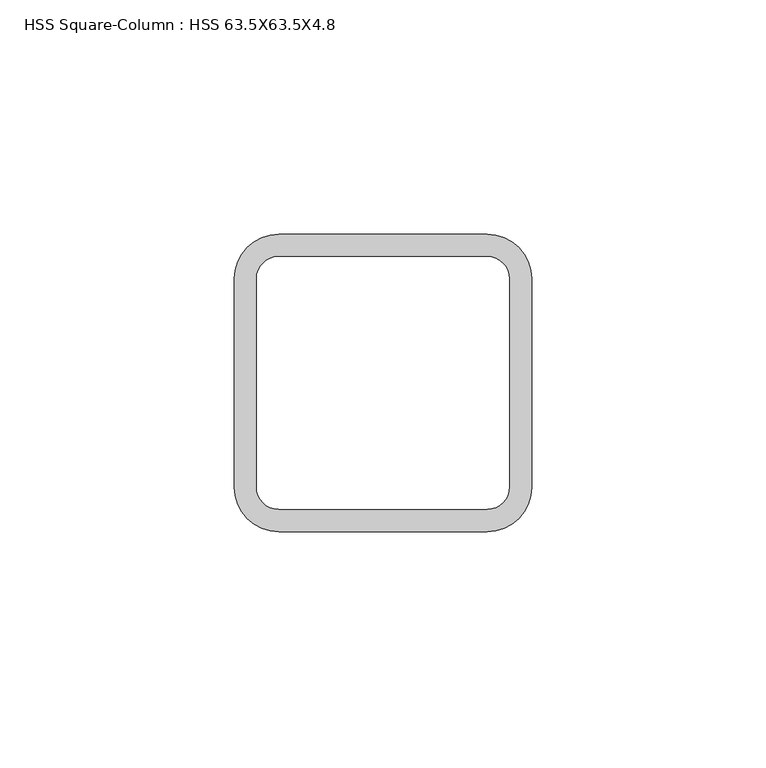
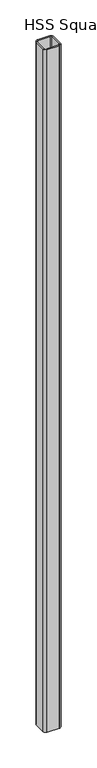
"""IFC4 building model written with IfcOpenShell, lengths in millimetres: column geometry, HSS Square-Column : HSS 63.5X63.5X4.8."""

from ifc_helpers import new_model, si_unit, point, frame, frame_2d, origin, place, context, project, spatial, polyline, circle_curve, trimmed, segment, composite_curve, outline, extrude, source, transform, mapped, element, save


def hss_square_column_hss_63_5x63_5x4_8_397be378(model_context):
    return source(origin(), model_context, "Body", "SweptSolid", [
        extrude(outline(composite_curve([segment(trimmed(circle_curve(frame_2d((22.225, 22.225)), 9.525), [point((22.225, 31.75))], [point((31.75, 22.225))], False, "CARTESIAN"), True, "CONTINUOUS"), segment(polyline([(31.75, 22.225), (31.75, -22.225)]), True, "CONTINUOUS"), segment(trimmed(circle_curve(frame_2d((22.225, -22.225)), 9.525), [point((31.75, -22.225))], [point((22.225, -31.75))], False, "CARTESIAN"), True, "CONTINUOUS"), segment(polyline([(22.225, -31.75), (-22.225, -31.75)]), True, "CONTINUOUS"), segment(trimmed(circle_curve(frame_2d((-22.225, -22.225)), 9.525), [point((-22.225, -31.75))], [point((-31.75, -22.225))], False, "CARTESIAN"), True, "CONTINUOUS"), segment(polyline([(-31.75, -22.225), (-31.75, 22.225)]), True, "CONTINUOUS"), segment(trimmed(circle_curve(frame_2d((-22.225, 22.225)), 9.525), [point((-31.75, 22.225))], [point((-22.225, 31.75))], False, "CARTESIAN"), True, "CONTINUOUS"), segment(polyline([(-22.225, 31.75), (22.225, 31.75)]), True, "CONTINUOUS")], self_intersect=False), holes=[composite_curve([segment(polyline([(22.225, 26.9875), (-22.225, 26.9875)]), True, "CONTINUOUS"), segment(trimmed(circle_curve(frame_2d((-22.225, 22.225)), 4.7625), [point((-22.225, 26.9875))], [point((-26.9875, 22.225))], True, "CARTESIAN"), True, "CONTINUOUS"), segment(polyline([(-26.9875, 22.225), (-26.9875, -22.225)]), True, "CONTINUOUS"), segment(trimmed(circle_curve(frame_2d((-22.225, -22.225)), 4.7625), [point((-26.9875, -22.225))], [point((-22.225, -26.9875))], True, "CARTESIAN"), True, "CONTINUOUS"), segment(polyline([(-22.225, -26.9875), (22.225, -26.9875)]), True, "CONTINUOUS"), segment(trimmed(circle_curve(frame_2d((22.225, -22.225)), 4.7625), [point((22.225, -26.9875))], [point((26.9875, -22.225))], True, "CARTESIAN"), True, "CONTINUOUS"), segment(polyline([(26.9875, -22.225), (26.9875, 22.225)]), True, "CONTINUOUS"), segment(trimmed(circle_curve(frame_2d((22.225, 22.225)), 4.7625), [point((26.9875, 22.225))], [point((22.225, 26.9875))], True, "CARTESIAN"), True, "CONTINUOUS")], self_intersect=False)]), frame((0.0, 0.0, 3220.0), z_axis=(0.0, 0.0, 1.0), x_axis=(1.0, 0.0, 0.0)), (0.0, 0.0, 1.0), 2650.0),
    ])


if __name__ == "__main__":
    model = new_model("IFC4")
    model_context = context("Model", 3, world=origin())
    ifc_project = project(units=[si_unit("LENGTHUNIT", "METRE", prefix="MILLI")], contexts=[model_context])
    site = spatial("IfcSite", under=ifc_project)
    building = spatial("IfcBuilding", under=site)
    placement = place(None, origin())
    hss_square_column_hss_63_5x63_5x4_8_shape = hss_square_column_hss_63_5x63_5x4_8_397be378(model_context)
    element("IfcColumn", 1, ObjectType="HSS Square-Column : HSS 63.5X63.5X4.8", at=placement, inside=building, context=model_context, shape_type="MappedRepresentation", body=[
        mapped(hss_square_column_hss_63_5x63_5x4_8_shape, transform((0.0, 0.0, 0.0), x_axis=(1.0, 0.0, 0.0), y_axis=(0.0, 1.0, 0.0), z_axis=(0.0, 0.0, 1.0))),
    ])
    save(model, "model.ifc")

# Revit data of these elements
# Type "HSS Square-Column : HSS 63.5X63.5X4.8"
#   Section Name Key = "HSS 2 1/2X2 1/2X3/16"
#   Assembly Code = "B10"
#   Width = 6.35 cm
#   Wall Nominal Thickness = 0.4763 cm
#   Wall Design Thickness = 0.442 cm
#   Torsional Moment of Inertia = 93.6521 cm⁴
#   Torsional Modulus = 30.4799 cm³
#   Section Area = 9.93546 cm²
#   Plastic Modulus weak axis = 21.6309 cm³
#   Plastic Modulus strong axis = 21.6309 cm³
#   Outer Fillet = 0.9525 cm
#   Nominal Weight = 8.31884 kgf/m
#   Moment of Inertia weak axis = 56.1912 cm⁴
#   Moment of Inertia strong axis = 56.1912 cm⁴
#   Inner Fillet = 0.4763 cm
#   Height = 6.35 cm
#   Elastic Modulus weak axis = 17.698 cm³
#   Elastic Modulus strong axis = 17.698 cm³
#   Centroid Vertical = 3.175 cm
#   Centroid Horizontal = 3.175 cm
#   Structural Material [instance default] = Steel ASTM A500, Grade B, Rectangular and Square
#   Principal Axes Angle = 0
# Element 1 (IfcColumn, "HSS Square-Column : HSS 63.5X63.5X4.8")
#   Structural Material = none
# Materials
#   "Steel ASTM A500, Grade B, Rectangular and Square": class "Metal", colour RGB 199 199 199, transparency 0, Description = "Carbon steel", Cost = 0
